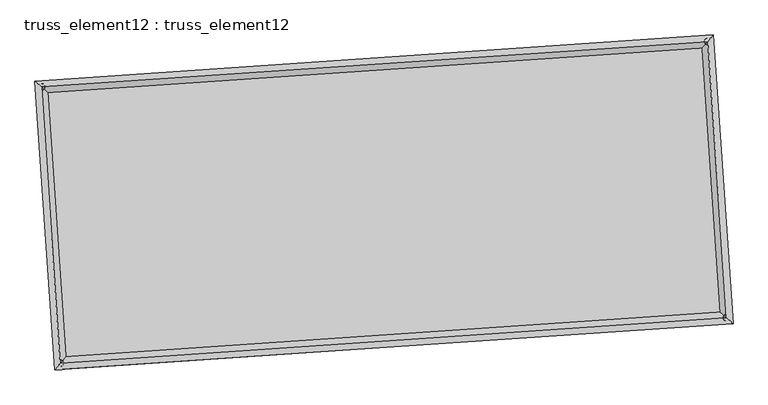
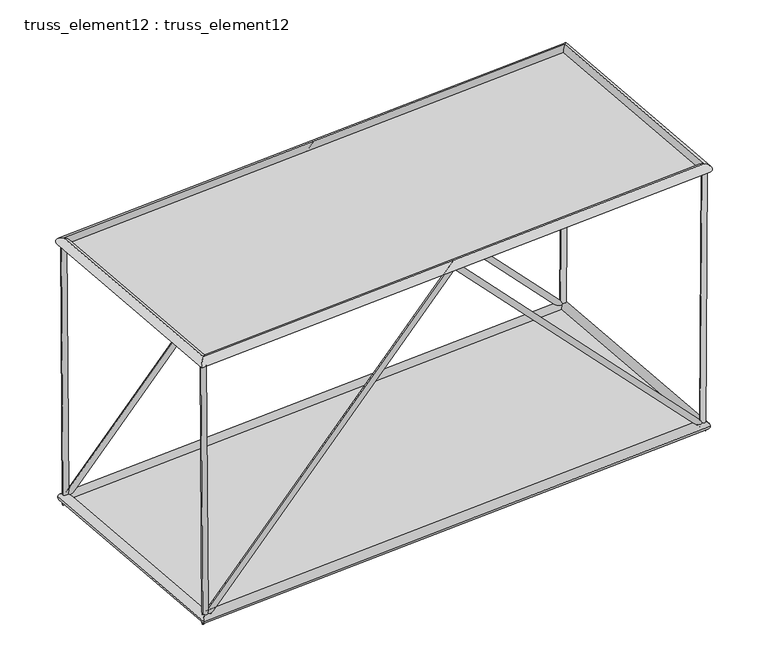
"""IFC4 building model written with IfcOpenShell, lengths in millimetres: plate geometry, truss_element12 : truss_element12."""

import ifcopenshell
import ifcopenshell.guid

model = None  # the IFC model being written
_history = None  # IfcOwnerHistory: only IFC2X3 demands one
_inside = {}  # id of a spatial element -> (the spatial element, [elements in it])
_under = {}  # id of a project, library or spatial element -> (it, [spatial elements below it])
_declared = {}  # id of a project -> (the project, [libraries it declares])
_typed = {}  # id of a type object -> (the type object, [elements of that type])
_made_of = {}  # id of a material, layer set ... -> (it, [elements and type objects made of it])


def new_model(schema):
    """Start an empty IFC model of exactly this schema.

    Asked for "IFC4X3", IfcOpenShell would pick the latest addendum, in which some entities
    have other attributes; the version numbers below select the first issue.
    IFC2X3 requires an IfcOwnerHistory on every rooted entity: one is made here for all.
    """
    global model, _history
    if schema == "IFC4X3":
        model = ifcopenshell.file(schema_version=(4, 3, 0, 0))
    else:
        model = ifcopenshell.file(schema=schema)
    _inside.clear()
    _under.clear()
    _declared.clear()
    _typed.clear()
    _made_of.clear()
    _history = None
    if model.schema == "IFC2X3":
        org = make("IfcOrganization", Name="unknown")
        user = make(
            "IfcPersonAndOrganization",
            ThePerson=make("IfcPerson", FamilyName="unknown"),
            TheOrganization=org,
        )
        app = make(
            "IfcApplication",
            ApplicationDeveloper=org,
            Version="unknown",
            ApplicationFullName="unknown",
            ApplicationIdentifier="unknown",
        )
        _history = make(
            "IfcOwnerHistory",
            OwningUser=user,
            OwningApplication=app,
            ChangeAction="ADDED",
            CreationDate=0,
        )
    return model


def make(cls, **values):
    """One entity of the class cls with the attributes given. An attribute that is None is left unset."""
    return model.create_entity(
        cls, **{name: value for name, value in values.items() if value is not None}
    )


def rooted(cls, **values):
    """An entity with a GlobalId (a new one), such as an element, a storey or a relation."""
    return make(cls, GlobalId=ifcopenshell.guid.new(), OwnerHistory=_history, **values)


def si_unit(unit_type, name, prefix=None):
    """IfcSIUnit, for example si_unit("LENGTHUNIT", "METRE", prefix="MILLI")."""
    return make("IfcSIUnit", UnitType=unit_type, Prefix=prefix, Name=name)


def assignment(units):
    """IfcUnitAssignment: the units of a project."""
    return None if units is None else make("IfcUnitAssignment", Units=units)


def point(xyz):
    """IfcCartesianPoint."""
    return None if xyz is None else make("IfcCartesianPoint", Coordinates=xyz)


def direction(xyz):
    """IfcDirection."""
    return None if xyz is None else make("IfcDirection", DirectionRatios=xyz)


def frame(location, z_axis=None, x_axis=None):
    """IfcAxis2Placement3D, a coordinate frame: its origin and axes. An axis left out is left unset."""
    return make(
        "IfcAxis2Placement3D",
        Location=point(location),
        Axis=direction(z_axis),
        RefDirection=direction(x_axis),
    )


def origin():
    """The frame at (0, 0, 0) with its axes left unset."""
    return frame((0.0, 0.0, 0.0))


def origin_with_axes():
    """The frame at (0, 0, 0) with the z axis (0, 0, 1) and the x axis (1, 0, 0) written out."""
    return frame((0.0, 0.0, 0.0), z_axis=(0.0, 0.0, 1.0), x_axis=(1.0, 0.0, 0.0))


def place(relative_to, where):
    """IfcLocalPlacement: puts the frame where relative to a parent placement (None: the world)."""
    return make(
        "IfcLocalPlacement", PlacementRelTo=relative_to, RelativePlacement=where
    )


def context(
    kind, dimensions, precision=None, world=None, true_north=None, identifier=None
):
    """IfcGeometricRepresentationContext, for example the 3D "Model" context."""
    return make(
        "IfcGeometricRepresentationContext",
        ContextIdentifier=identifier,
        ContextType=kind,
        CoordinateSpaceDimension=dimensions,
        Precision=precision,
        WorldCoordinateSystem=world,
        TrueNorth=true_north,
    )


def project(units=None, contexts=None):
    """IfcProject with its units and contexts."""
    return rooted(
        "IfcProject",
        Name="project",
        RepresentationContexts=contexts,
        UnitsInContext=assignment(units),
    )


def spatial(cls, under=None, at=None, **own):
    """A site, building, storey or space (cls), placed at a placement, below another one or the project."""
    s = rooted(cls, ObjectPlacement=at, **own)
    if under is not None:
        _under.setdefault(under.id(), (under, []))[1].append(s)
    return s


def polyline(points):
    """IfcPolyline through the points."""
    return make("IfcPolyline", Points=[point(p) for p in points])


def circle_curve(where, radius):
    """IfcCircle in the frame where."""
    return make("IfcCircle", Position=where, Radius=radius)


def ellipse_curve(where, semi_axis1, semi_axis2):
    """IfcEllipse in the frame where."""
    return make(
        "IfcEllipse", Position=where, SemiAxis1=semi_axis1, SemiAxis2=semi_axis2
    )


def outline(outer, holes=None, kind="AREA"):
    """IfcArbitraryClosedProfileDef: a profile drawn as a closed curve; with holes, ...WithVoids."""
    if holes is None:
        return make("IfcArbitraryClosedProfileDef", ProfileType=kind, OuterCurve=outer)
    return make(
        "IfcArbitraryProfileDefWithVoids",
        ProfileType=kind,
        OuterCurve=outer,
        InnerCurves=holes,
    )


def extrude(swept, where, along, depth):
    """IfcExtrudedAreaSolid: the profile swept, set in the frame where, extruded along a direction by depth."""
    return make(
        "IfcExtrudedAreaSolid",
        SweptArea=swept,
        Position=where,
        ExtrudedDirection=direction(along),
        Depth=depth,
    )


def shape(context_of_items, identifier, shape_type, items):
    """IfcShapeRepresentation: the items that make up one representation, for example the "Body"."""
    return make(
        "IfcShapeRepresentation",
        ContextOfItems=context_of_items,
        RepresentationIdentifier=identifier,
        RepresentationType=shape_type,
        Items=items,
    )


def source(mapping_origin, context_of_items, identifier, shape_type, items):
    """IfcRepresentationMap: a shape defined once, which mapped items show again and again."""
    return make(
        "IfcRepresentationMap",
        MappingOrigin=mapping_origin,
        MappedRepresentation=shape(context_of_items, identifier, shape_type, items),
    )


def transform(
    local_origin,
    x_axis=None,
    y_axis=None,
    z_axis=None,
    scale=None,
    scale2=None,
    scale3=None,
    uniform=True,
):
    """IfcCartesianTransformationOperator3D, or its non-uniform kind. x_axis, y_axis, z_axis: its Axis1, 2, 3."""
    if uniform:
        return make(
            "IfcCartesianTransformationOperator3D",
            Axis1=direction(x_axis),
            Axis2=direction(y_axis),
            LocalOrigin=point(local_origin),
            Scale=scale,
            Axis3=direction(z_axis),
        )
    return make(
        "IfcCartesianTransformationOperator3DnonUniform",
        Axis1=direction(x_axis),
        Axis2=direction(y_axis),
        LocalOrigin=point(local_origin),
        Scale=scale,
        Axis3=direction(z_axis),
        Scale2=scale2,
        Scale3=scale3,
    )


def mapped(mapping_source, mapping_target):
    """IfcMappedItem: shows the shape of a source again, moved by a transform."""
    return make(
        "IfcMappedItem", MappingSource=mapping_source, MappingTarget=mapping_target
    )


def made_of(thing, what):
    """Note that an element or type object is made of a material, layer set ...; save() writes the relation."""
    if what is not None:
        _made_of.setdefault(what.id(), (what, []))[1].append(thing)
    return thing


def element(
    cls,
    number,
    at=None,
    inside=None,
    cuts=None,
    type_object=None,
    material=None,
    context=None,
    identifier="Body",
    shape_type=None,
    held_by="IfcProductDefinitionShape",
    body=None,
    shapes=None,
    **own,
):
    """One element of the class cls, such as IfcWall. Its Tag is "e" and its number.

    at: its placement. inside: the storey or other place that contains it. cuts: it is an
    opening in that element (IfcRelVoidsElement). A single representation is given by context,
    identifier, shape_type and body (its items); several are given by shapes. held_by: the class
    of the entity that holds the representations. save() writes the other relations.
    """
    e = rooted(cls, Tag="e%d" % number, ObjectPlacement=at, **own)
    if body is not None:
        shapes = [shape(context, identifier, shape_type, body)]
    if shapes is not None:
        e.Representation = make(held_by, Representations=shapes)
    if inside is not None:
        _inside.setdefault(inside.id(), (inside, []))[1].append(e)
    if cuts is not None:
        rooted(
            "IfcRelVoidsElement", RelatingBuildingElement=cuts, RelatedOpeningElement=e
        )
    if type_object is not None:
        _typed.setdefault(type_object.id(), (type_object, []))[1].append(e)
    return made_of(e, material)


def aggregate(whole, parts):
    """IfcRelAggregates: a whole, such as a stair, and the parts it consists of."""
    return rooted("IfcRelAggregates", RelatingObject=whole, RelatedObjects=parts)


def save(model, path):
    """Write the relations noted so far, then the file.

    IfcRelAggregates (storeys below a building ...), IfcRelContainedInSpatialStructure (elements
    in a storey), IfcRelDefinesByType, IfcRelAssociatesMaterial and IfcRelDeclares: one each for
    every whole, place, type object, material and project.
    """
    for whole, parts in _under.values():
        aggregate(whole, parts)
    for where, things in _inside.values():
        rooted(
            "IfcRelContainedInSpatialStructure",
            RelatedElements=things,
            RelatingStructure=where,
        )
    for kind, things in _typed.values():
        rooted("IfcRelDefinesByType", RelatedObjects=things, RelatingType=kind)
    for what, things in _made_of.values():
        rooted("IfcRelAssociatesMaterial", RelatedObjects=things, RelatingMaterial=what)
    for by, libraries in _declared.values():
        rooted("IfcRelDeclares", RelatingContext=by, RelatedDefinitions=libraries)
    model.write(path)


def plane_surface(at):
    """IfcPlane: the flat surface through the origin of the frame at, square to its z axis."""
    return make("IfcPlane", Position=at)


def cylinder_surface(at, radius):
    """IfcCylindricalSurface: all points at the distance radius from the z axis of the frame at."""
    return make("IfcCylindricalSurface", Position=at, Radius=radius)


def advanced_brep(points, edges, surfaces, faces):
    """IfcAdvancedBrep: a solid bounded by faces that lie on surfaces and meet in shared edges.

    An edge is (start, end): straight between two places in points (the first is 0);
    or (start, end, curve); or (start, end, curve, False) where it runs against its curve.
    A face is (place in surfaces, loops), or (place, loops, False) where it looks against
    its surface's normal. A loop lists edges by number (the first is 1), with a minus sign
    where the edge is run from its end to its start. The first loop is the outer one.
    """
    corners = [point(p) for p in points]
    vertices = [make("IfcVertexPoint", VertexGeometry=c) for c in corners]
    made = []
    for start, end, *more in edges:
        made.append(
            make(
                "IfcEdgeCurve",
                EdgeStart=vertices[start],
                EdgeEnd=vertices[end],
                EdgeGeometry=more[0] if more else make("IfcPolyline", Points=[corners[start], corners[end]]),
                SameSense=more[1] if len(more) > 1 else True,
            )
        )
    hull = []
    for where, loops, *sense in faces:
        bounds = []
        for j, loop in enumerate(loops):
            ring = [make("IfcOrientedEdge", EdgeElement=made[abs(k) - 1], Orientation=k > 0) for k in loop]
            bounds.append(
                make(
                    "IfcFaceOuterBound" if j == 0 else "IfcFaceBound",
                    Bound=make("IfcEdgeLoop", EdgeList=ring),
                    Orientation=True,
                )
            )
        hull.append(make("IfcAdvancedFace", Bounds=bounds, FaceSurface=surfaces[where], SameSense=sense[0] if sense else True))
    return make("IfcAdvancedBrep", Outer=make("IfcClosedShell", CfsFaces=hull))


def truss_element12_truss_element12_0bdd8d05(model_context):
    return source(origin(), model_context, "Body", "SolidModel", [
        advanced_brep(
        [(-3699.2780171, 2273.8827184, 5000.224961), (-3798.3790208, 2260.5216048, 4999.5381605), (-3665.7874801, 2276.1663109, 123.3255888), (-3763.1994027, 2262.9203692, -123.3255888), (1063.4543836, 2598.635336, 5072.0064394), (1063.9065449, 2592.0623743, 4927.760284), (5793.213407, 2921.1396243, 123.3293252), (5891.54757, 2921.2408642, -123.3293252), (5826.190706, 2923.388221, 5000.223301), (5926.1881888, 2923.6028763, 4999.5470243)],
        [
            (0, 1, circle_curve(frame((-3748.828519, 2267.2021616, 4999.8815607), z_axis=(-0.006867015509295821, -0.000468235683609246, 0.9999763121461127), x_axis=(-0.13361118718071577, 0.9910337254669442, -0.0004534834827120485)), 50.0)),
            (1, 0, circle_curve(frame((-3748.828519, 2267.2021616, 4999.8815607), z_axis=(-0.006867015509295821, -0.000468235683609246, 0.9999763121461127), x_axis=(-0.13361118718071577, 0.9910337254669442, -0.0004534834827120485)), 50.0)),
            (0, 2),
            (2, 3, ellipse_curve(frame((-3714.4934414, 2269.54334, 0.0), z_axis=(-0.927066716557074, -0.06321315529151074, 0.3695286187160306), x_axis=(0.3686725672674677, 0.025138380906336275, 0.9292193497500052)), 133.0085635, 50.0)),
            (3, 1),
            (3, 2, ellipse_curve(frame((-3714.4934414, 2269.54334, 0.0), z_axis=(-0.927066716557074, -0.06321315529151074, 0.3695286187160306), x_axis=(0.3686725672674677, 0.025138380906336275, 0.9292193497500052)), 133.0085635, 50.0)),
            (2, 4),
            (4, 5, ellipse_curve(frame((1063.6804642, 2595.3488551, 4999.8833617), z_axis=(-0.9976833956976204, -0.06802823820297604, -2.750026008393468e-05), x_axis=(2.7436552873218184e-05, 1.8707942446141108e-06, -0.9999999996218679)), 72.2801261, 50.0)),
            (5, 3),
            (5, 4, ellipse_curve(frame((1063.6804642, 2595.3488551, 4999.8833617), z_axis=(-0.9976833956976204, -0.06802823820297604, -2.750026008393468e-05), x_axis=(2.7436552873218184e-05, 1.8707942446141108e-06, -0.9999999996218679)), 72.2801261, 50.0)),
            (4, 6),
            (6, 7, ellipse_curve(frame((5842.3804885, 2921.1902443, 0.0), z_axis=(-0.9270371329382554, -0.06321113809700134, -0.3696031739231976), x_axis=(-0.368746949759749, -0.025143452765731062, 0.9291896974385255)), 133.0168379, 50.0)),
            (7, 5),
            (7, 6, ellipse_curve(frame((5842.3804885, 2921.1902443, 0.0), z_axis=(-0.9270371329382554, -0.06321113809700134, -0.3696031739231976), x_axis=(-0.368746949759749, -0.025143452765731062, 0.9291896974385255)), 133.0168379, 50.0)),
            (8, 9, circle_curve(frame((5876.1894474, 2923.4955486, 4999.8851627), z_axis=(0.006761791779643145, 0.0004610608774766411, 0.9999770325336459), x_axis=(-0.002149622020133885, 0.9999975898630503, -0.00044653472552298745)), 50.0)),
            (9, 8, circle_curve(frame((5876.1894474, 2923.4955486, 4999.8851627), z_axis=(0.006761791779643145, 0.0004610608774766411, 0.9999770325336459), x_axis=(-0.002149622020133885, 0.9999975898630503, -0.00044653472552298745)), 50.0)),
            (6, 8),
            (9, 7),
        ],
        [
            plane_surface(frame((-3748.828519, 2317.2021561, 4999.9049731), z_axis=(-0.006867015509297537, -0.0004682356836103226, 0.9999763121461126), x_axis=(0.9999764217710311, -3.215457516247967e-06, 0.006867014756483772))),
            cylinder_surface(frame((-3748.828519, 2267.2021616, 4999.8815607), z_axis=(-0.006867015509295821, -0.000468235683609246, 0.9999763121461127), x_axis=(-0.13361118718071577, 0.9910337254669442, -0.0004534834827120485)), 50.0),
            cylinder_surface(frame((-3714.4934414, 2269.54334, 0.0), z_axis=(-0.6901307509390465, -0.04705739247394388, -0.7221531336370847), x_axis=(-0.0204116303240351, 0.9987523729372, -0.04557480553800632)), 50.0),
            cylinder_surface(frame((1063.6804642, 2595.3488551, 4999.8833617), z_axis=(-0.6901703766804564, -0.04706009440261949, 0.7221150868577483), x_axis=(-0.11534672532663481, 0.9922791096910546, -0.04557742233990455)), 50.0),
            plane_surface(frame((5876.1894474, 2873.495554, 4999.9082162), z_axis=(0.006761791779644185, 0.00046106087747216243, 0.9999770325336457), x_axis=(0.9999771388246477, -3.1176689248013658e-06, -0.00676179106091013))),
            cylinder_surface(frame((5842.3804885, 2921.1902443, 0.0), z_axis=(-0.006761791779643143, -0.000461060877476641, -0.9999770325336457), x_axis=(-0.002149622020133885, 0.9999975898630503, -0.00044653472552298745)), 50.0),
        ],
        [
            (0, [[1, 2]]),
            (1, [[-1, 3, 4, 5]]),
            (1, [[-2, -5, 6, -3]]),
            (2, [[-4, 7, 8, 9]]),
            (2, [[-6, -9, 10, -7]]),
            (3, [[-8, 11, 12, 13]]),
            (3, [[-10, -13, 14, -11]]),
            (4, [[15, 16]]),
            (5, [[-12, 17, -16, 18]]),
            (5, [[-14, -18, -15, -17]]),
        ],
    ),
        advanced_brep(
        [(-3427.1650642, -1716.8508659, 5000.224961), (-3526.2660679, -1730.2119795, 4999.5381605), (-3393.6745272, -1714.5672734, 123.3255888), (-3491.0864498, -1727.8132151, -123.3255888), (1335.5673365, -1392.0982483, 5072.0064394), (1336.0194978, -1398.67121, 4927.760284), (6065.3263599, -1069.59396, 123.3293252), (6163.6605229, -1069.4927201, -123.3293252), (6098.3036589, -1067.3453633, 5000.223301), (6198.3011417, -1067.130708, 4999.5470243)],
        [
            (0, 1, circle_curve(frame((-3476.715566, -1723.5314227, 4999.8815607), z_axis=(-0.006867015509295706, -0.0004682356836092419, 0.9999763121461127), x_axis=(-0.13361118718071638, 0.9910337254669442, -0.0004534834827120414)), 50.0)),
            (1, 0, circle_curve(frame((-3476.715566, -1723.5314227, 4999.8815607), z_axis=(-0.006867015509295706, -0.0004682356836092419, 0.9999763121461127), x_axis=(-0.13361118718071638, 0.9910337254669442, -0.0004534834827120414)), 50.0)),
            (0, 2),
            (2, 3, ellipse_curve(frame((-3442.3804885, -1721.1902443, 0.0), z_axis=(-0.9270667165570737, -0.06321315529151104, 0.36952861871603054), x_axis=(0.36867256726746755, 0.02513838090633639, 0.9292193497500053)), 133.0085635, 50.0)),
            (3, 1),
            (3, 2, ellipse_curve(frame((-3442.3804885, -1721.1902443, 0.0), z_axis=(-0.9270667165570737, -0.06321315529151104, 0.36952861871603054), x_axis=(0.36867256726746755, 0.02513838090633639, 0.9292193497500053)), 133.0085635, 50.0)),
            (2, 4),
            (4, 5, ellipse_curve(frame((1335.7934171, -1395.3847292, 4999.8833617), z_axis=(-0.9976833956976204, -0.06802823820297628, -2.750026008401492e-05), x_axis=(2.743655287337192e-05, 1.8707942445372394e-06, -0.9999999996218679)), 72.2801261, 50.0)),
            (5, 3),
            (5, 4, ellipse_curve(frame((1335.7934171, -1395.3847292, 4999.8833617), z_axis=(-0.9976833956976204, -0.06802823820297628, -2.750026008401492e-05), x_axis=(2.743655287337192e-05, 1.8707942445372394e-06, -0.9999999996218679)), 72.2801261, 50.0)),
            (4, 6),
            (6, 7, ellipse_curve(frame((6114.4934414, -1069.54334, 0.0), z_axis=(-0.9270371329382552, -0.06321113809700153, -0.3696031739231974), x_axis=(-0.368746949759749, -0.025143452765731107, 0.9291896974385254)), 133.0168379, 50.0)),
            (7, 5),
            (7, 6, ellipse_curve(frame((6114.4934414, -1069.54334, 0.0), z_axis=(-0.9270371329382552, -0.06321113809700153, -0.3696031739231974), x_axis=(-0.368746949759749, -0.025143452765731107, 0.9291896974385254)), 133.0168379, 50.0)),
            (8, 9, circle_curve(frame((6148.3024003, -1067.2380357, 4999.8851627), z_axis=(0.006761791779642977, 0.0004610608774766668, 0.9999770325336459), x_axis=(-0.002149622020133642, 0.9999975898630503, -0.00044653472552301515)), 50.0)),
            (9, 8, circle_curve(frame((6148.3024003, -1067.2380357, 4999.8851627), z_axis=(0.006761791779642977, 0.0004610608774766668, 0.9999770325336459), x_axis=(-0.002149622020133642, 0.9999975898630503, -0.00044653472552301515)), 50.0)),
            (6, 8),
            (9, 7),
        ],
        [
            plane_surface(frame((-3476.715566, -1673.5314282, 4999.9049731), z_axis=(-0.006867015509297537, -0.0004682356836103226, 0.9999763121461126), x_axis=(0.9999764217710311, -3.215457516247967e-06, 0.006867014756483772))),
            cylinder_surface(frame((-3476.715566, -1723.5314227, 4999.8815607), z_axis=(-0.006867015509295706, -0.0004682356836092419, 0.9999763121461127), x_axis=(-0.13361118718071638, 0.9910337254669442, -0.0004534834827120414)), 50.0),
            cylinder_surface(frame((-3442.3804885, -1721.1902443, 0.0), z_axis=(-0.6901307509390463, -0.04705739247394409, -0.7221531336370847), x_axis=(-0.020411630324035174, 0.9987523729372, -0.04557480553800655)), 50.0),
            cylinder_surface(frame((1335.7934171, -1395.3847292, 4999.8833617), z_axis=(-0.6901703766804567, -0.04706009440261962, 0.7221150868577483), x_axis=(-0.1153467253266352, 0.9922791096910545, -0.04557742233990476)), 50.0),
            plane_surface(frame((6148.3024003, -1117.2380303, 4999.9082162), z_axis=(0.006761791779644185, 0.0004610608774721631, 0.9999770325336457), x_axis=(0.9999771388246477, -3.1176689248013658e-06, -0.00676179106091013))),
            cylinder_surface(frame((6114.4934414, -1069.54334, 0.0), z_axis=(-0.006761791779642976, -0.0004610608774766667, -0.9999770325336457), x_axis=(-0.002149622020133642, 0.9999975898630503, -0.00044653472552301515)), 50.0),
        ],
        [
            (0, [[1, 2]]),
            (1, [[-1, 3, 4, 5]]),
            (1, [[-2, -5, 6, -3]]),
            (2, [[-4, 7, 8, 9]]),
            (2, [[-6, -9, 10, -7]]),
            (3, [[-8, 11, 12, 13]]),
            (3, [[-10, -13, 14, -11]]),
            (4, [[15, 16]]),
            (5, [[-12, 17, -16, 18]]),
            (5, [[-14, -18, -15, -17]]),
        ],
    ),
        advanced_brep(
        [(-3476.7146152, -1723.5303688, 4909.8815607), (-3476.7165169, -1723.5324765, 5089.8815607), (-3748.8296041, 2267.2030767, 5089.8815607), (-3748.8274338, 2267.2012466, 4909.8815607), (5876.1903312, 2923.4965979, 5089.8851627), (5876.1885636, 2923.4944993, 4909.8851627), (6148.3034184, -1067.2389553, 5089.8851627), (6148.3013822, -1067.237116, 4909.8851627)],
        [
            (0, 1, ellipse_curve(frame((-3476.715566, -1723.5314227, 4999.8815607), z_axis=(-0.7535719234054068, 0.6573654662780862, -2.6400514555865953e-07), x_axis=(-0.6573654662780336, -0.7535719234054529, -2.640051451758168e-07)), 127.2792206, 90.0)),
            (1, 2),
            (2, 3, ellipse_curve(frame((-3748.828519, 2267.2021616, 4999.8815607), z_axis=(-0.6573654662780338, -0.7535719234054528, -2.6400514525519494e-07), x_axis=(0.7535719234054069, -0.6573654662780862, 2.640051456380377e-07)), 127.2792206, 90.0)),
            (3, 0),
            (1, 0, ellipse_curve(frame((-3476.715566, -1723.5314227, 4999.8815607), z_axis=(-0.7535719234054068, 0.6573654662780862, -2.6400514555865953e-07), x_axis=(-0.6573654662780336, -0.7535719234054529, -2.640051451758168e-07)), 127.2792206, 90.0)),
            (3, 2, ellipse_curve(frame((-3748.828519, 2267.2021616, 4999.8815607), z_axis=(-0.6573654662780338, -0.7535719234054528, -2.6400514525519494e-07), x_axis=(0.7535719234054069, -0.6573654662780862, 2.640051456380377e-07)), 127.2792206, 90.0)),
            (2, 4),
            (4, 5, ellipse_curve(frame((5876.1894474, 2923.4955486, 4999.8851627), z_axis=(-0.7535719234054068, 0.6573654662780863, -2.6400514544662063e-07), x_axis=(-0.6573654662780339, -0.7535719234054526, -2.6400514544661195e-07)), 127.2792206, 90.0)),
            (5, 3),
            (5, 4, ellipse_curve(frame((5876.1894474, 2923.4955486, 4999.8851627), z_axis=(-0.7535719234054068, 0.6573654662780863, -2.6400514544662063e-07), x_axis=(-0.6573654662780339, -0.7535719234054526, -2.6400514544661195e-07)), 127.2792206, 90.0)),
            (4, 6),
            (6, 7, ellipse_curve(frame((6148.3024003, -1067.2380357, 4999.8851627), z_axis=(0.6573654662780338, 0.7535719234054526, 2.6400514536723384e-07), x_axis=(-0.7535719234054067, 0.6573654662780865, -2.640051453672425e-07)), 127.2792206, 90.0)),
            (7, 5),
            (7, 6, ellipse_curve(frame((6148.3024003, -1067.2380357, 4999.8851627), z_axis=(0.6573654662780338, 0.7535719234054526, 2.6400514536723384e-07), x_axis=(-0.7535719234054067, 0.6573654662780865, -2.640051453672425e-07)), 127.2792206, 90.0)),
            (6, 1),
            (0, 7),
        ],
        [
            cylinder_surface(frame((-3476.715566, -1723.5314227, 4999.8815607), z_axis=(0.0680282382286978, -0.9976833960748769, 0.0), x_axis=(-0.9976833960107591, -0.06802823822432585, -1.1337253580804916e-05)), 90.0),
            cylinder_surface(frame((-3748.828519, 2267.2021616, 4999.8815607), z_axis=(-0.9976833960748073, -0.06802823822869414, -3.7335965722688633e-07), x_axis=(-0.06802823822052616, 0.997683396015191, -1.0963893923871191e-05)), 90.0),
            cylinder_surface(frame((5876.1894474, 2923.4955486, 4999.8851627), z_axis=(-0.06802823822869772, 0.9976833960748769, 0.0), x_axis=(0.9976833960189271, 0.06802823822488271, -1.0590534266666754e-05)), 90.0),
            cylinder_surface(frame((6148.3024003, -1067.2380357, 4999.8851627), z_axis=(0.9976833960748072, 0.06802823822869412, 3.733596571146287e-07), x_axis=(0.06802823822869412, -0.997683396014634, -1.0963893923758946e-05)), 90.0),
        ],
        [
            (0, [[1, 2, 3, 4]]),
            (0, [[5, -4, 6, -2]]),
            (1, [[-3, 7, 8, 9]]),
            (1, [[-6, -9, 10, -7]]),
            (2, [[-8, 11, 12, 13]]),
            (2, [[-10, -13, 14, -11]]),
            (3, [[-12, 15, -1, 16]]),
            (3, [[-14, -16, -5, -15]]),
        ],
    ),
        advanced_brep(
        [(-3358.7115243, -1625.2761972, 0.0), (-3526.0494527, -1817.1042913, 0.0), (-3810.4074885, 2353.2123043, 0.0), (-3618.5793943, 2185.8743758, 0.0), (5926.0494527, 3017.1042913, 0.0), (5758.7115243, 2825.2761972, 0.0), (6210.4074885, -1153.2123043, 0.0), (6018.5793943, -985.8743758, 0.0)],
        [
            (0, 1, ellipse_curve(frame((-3442.3804885, -1721.1902443, 0.0), z_axis=(-0.7535719234054564, 0.6573654662780825, 0.0), x_axis=(-0.6573654662780822, -0.7535719234054566, 0.0)), 127.2792206, 90.0)),
            (1, 2),
            (2, 3, ellipse_curve(frame((-3714.4934414, 2269.54334, 0.0), z_axis=(-0.6573654662780825, -0.7535719234054565, 0.0), x_axis=(0.7535719234054564, -0.6573654662780825, 0.0)), 127.2792206, 90.0)),
            (3, 0),
            (1, 0, ellipse_curve(frame((-3442.3804885, -1721.1902443, 0.0), z_axis=(-0.7535719234054564, 0.6573654662780825, 0.0), x_axis=(-0.6573654662780822, -0.7535719234054566, 0.0)), 127.2792206, 90.0)),
            (3, 2, ellipse_curve(frame((-3714.4934414, 2269.54334, 0.0), z_axis=(-0.6573654662780825, -0.7535719234054565, 0.0), x_axis=(0.7535719234054564, -0.6573654662780825, 0.0)), 127.2792206, 90.0)),
            (2, 4),
            (4, 5, ellipse_curve(frame((5842.3804885, 2921.1902443, 0.0), z_axis=(-0.7535719234054564, 0.6573654662780825, 0.0), x_axis=(-0.6573654662780826, -0.7535719234054563, 0.0)), 127.2792206, 90.0)),
            (5, 3),
            (5, 4, ellipse_curve(frame((5842.3804885, 2921.1902443, 0.0), z_axis=(-0.7535719234054564, 0.6573654662780825, 0.0), x_axis=(-0.6573654662780826, -0.7535719234054563, 0.0)), 127.2792206, 90.0)),
            (4, 6),
            (6, 7, ellipse_curve(frame((6114.4934414, -1069.54334, 0.0), z_axis=(0.6573654662780827, 0.7535719234054565, 0.0), x_axis=(-0.7535719234054566, 0.6573654662780823, 0.0)), 127.2792206, 90.0)),
            (7, 5),
            (7, 6, ellipse_curve(frame((6114.4934414, -1069.54334, 0.0), z_axis=(0.6573654662780827, 0.7535719234054565, 0.0), x_axis=(-0.7535719234054566, 0.6573654662780823, 0.0)), 127.2792206, 90.0)),
            (6, 1),
            (0, 7),
        ],
        [
            cylinder_surface(frame((-3442.3804885, -1721.1902443, 0.0), z_axis=(0.0680282382286986, -0.9976833960748768, 0.0), x_axis=(-0.9976833960748768, -0.0680282382286986, 0.0)), 90.0),
            cylinder_surface(frame((-3714.4934414, 2269.54334, 0.0), z_axis=(-0.9976833960748768, -0.06802823822869966, 0.0), x_axis=(-0.06802823822869966, 0.9976833960748768, 0.0)), 90.0),
            cylinder_surface(frame((5842.3804885, 2921.1902443, 0.0), z_axis=(-0.06802823822869838, 0.9976833960748769, 0.0), x_axis=(0.9976833960748769, 0.06802823822869838, 0.0)), 90.0),
            cylinder_surface(frame((6114.4934414, -1069.54334, 0.0), z_axis=(0.9976833960748768, 0.06802823822869936, 0.0), x_axis=(0.06802823822869936, -0.9976833960748768, 0.0)), 90.0),
        ],
        [
            (0, [[1, 2, 3, 4]]),
            (0, [[5, -4, 6, -2]]),
            (1, [[-3, 7, 8, 9]]),
            (1, [[-6, -9, 10, -7]]),
            (2, [[-8, 11, 12, 13]]),
            (2, [[-10, -13, 14, -11]]),
            (3, [[-12, 15, -1, 16]]),
            (3, [[-14, -16, -5, -15]]),
        ],
    ),
        extrude(outline(polyline([(-3442.3804885, -1721.1902443), (-3714.4934414, 2269.54334), (5842.3804885, 2921.1902443), (6114.4934414, -1069.54334), (-3442.3804885, -1721.1902443)])), origin_with_axes(), (0.0, 0.0, 1.0), 20.0),
        extrude(outline(polyline([(-2000.0, 4823.6835474), (2000.0, 4823.6835475), (1999.9999999, -4823.6835474), (-2000.0000001, -4823.6835474), (-2000.0, 4823.6835474)])), frame((1199.7369407, 599.982063, 4999.8833617), z_axis=(-3.72494730797882e-07, -2.539899943672577e-08, 0.9999999999999304), x_axis=(-0.06802823822869852, 0.9976833960748768, 0.0)), (0.0, 0.0, 1.0), 20.0),
    ])


if __name__ == "__main__":
    model = new_model("IFC4")
    model_context = context("Model", 3, world=origin())
    ifc_project = project(units=[si_unit("LENGTHUNIT", "METRE", prefix="MILLI")], contexts=[model_context])
    site = spatial("IfcSite", under=ifc_project)
    building = spatial("IfcBuilding", under=site)
    placement = place(None, origin())
    truss_element12_truss_element12_shape = truss_element12_truss_element12_0bdd8d05(model_context)
    element("IfcPlate", 1, ObjectType="truss_element12 : truss_element12", at=placement, inside=building, context=model_context, shape_type="MappedRepresentation", body=[
        mapped(truss_element12_truss_element12_shape, transform((0.0, 0.0, 0.0), x_axis=(1.0, 0.0, 0.0), y_axis=(0.0, 1.0, 0.0), z_axis=(0.0, 0.0, 1.0))),
    ])
    save(model, "model.ifc")

# Revit data of these elements
# Project information
#   Project Issue Date = "Issue Date"
#   Project Status = "Project Status"
#   Client Name = "Owner"
#   Project Address = "Enter address here"
#   Project Name = "Project Name"
#   Project Number = "Project Number"
# Type "truss_element12 : truss_element12"
#   steellbar1 = 90 mm
#   steelbar2 = 50 mm
#   offset1 = 5000 mm
#   M = Default Roof
# Element 1 (IfcPlate, "truss_element12 : truss_element12")
#   Materials on its faces: "Default Roof"
# Materials
#   "Default Roof": class "Miscellaneous", colour RGB 0 127 0, transparency 0, Comments = "Rendering appearance not upgraded Rendering appearance not upgraded ", Cost = 0
